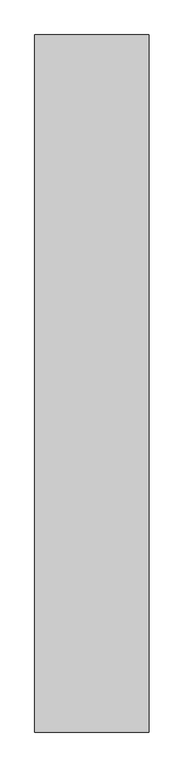
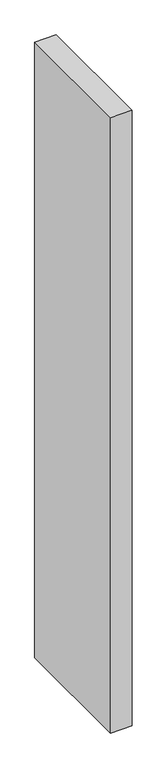
"""IFC4 building model written with IfcOpenShell, lengths in millimetres: proxy geometry, Generic Models 7:Generic Models 1:3:Generic Models 1:3 : Generic Models 7:Generic Models 1:305549:3:Generic Models 1:3:Generic Models 1:3 : Generic Models 7:Generic Models 1:305549:3 : Generic Models 7:Generic Models 1:3:Generic Models 1:3 : Generic Models 7:Generic Models 1:305549:301244:51 : Generic Models 7:Generic Models 1:3:Generic Models 1:3 : Generic Models 7:Generic Models 1:305549:3:Generic Models 1:3:Generic Models 1:3 : Generic Models 7:Generic Models 1:305549:3 : Generic Models 7:Generic Models 1:3:Generic Models 1:3 : Generic Models 7:Generic Models 1:305549:301244:308848."""

from ifc_helpers import new_model, si_unit, origin, origin_with_axes, place, context, project, spatial, polyline, outline, extrude, source, transform, mapped, element, save


def generic_models_49c228d4(model_context):
    return source(origin(), model_context, "Body", "SweptSolid", [
        extrude(outline(polyline([(667344.1117239, -569445.8514763), (667344.1117239, -568206.287148), (667547.3117239, -568206.287148), (667547.3117239, -569445.8514763), (667344.1117239, -569445.8514763)])), origin_with_axes(), (0.0, 0.0, 1.0), 6127.75),
    ])


if __name__ == "__main__":
    model = new_model("IFC4")
    model_context = context("Model", 3, world=origin())
    ifc_project = project(units=[si_unit("LENGTHUNIT", "METRE", prefix="MILLI")], contexts=[model_context])
    site = spatial("IfcSite", under=ifc_project)
    building = spatial("IfcBuilding", under=site)
    placement = place(None, origin())
    generic_models_shape = generic_models_49c228d4(model_context)
    element("IfcBuildingElementProxy", 1, Name="Generic Models 7:Generic Models 1:3:Generic Models 1:3 : Generic Models 7:Generic Models 1:305549:3:Generic Models 1:3:Generic Models 1:3 : Generic Models 7:Generic Models 1:305549:3 : Generic Models 7:Generic Models 1:3:Generic Models 1:3 : Generic Models 7:Generic Models 1:305549:301244:51 : Generic Models 7:Generic Models 1:3:Generic Models 1:3 : Generic Models 7:Generic Models 1:305549:3:Generic Models 1:3:Generic Models 1:3 : Generic Models 7:Generic Models 1:305549:3 : Generic Models 7:Generic Models 1:3:Generic Models 1:3 : Generic Models 7:Generic Models 1:305549:301244:308848", ObjectType="Generic Models 7:Generic Models 1:3:Generic Models 1:3 : Generic Models 7:Generic Models 1:305549:3:Generic Models 1:3:Generic Models 1:3 : Generic Models 7:Generic Models 1:305549:3 : Generic Models 7:Generic Models 1:3:Generic Models 1:3 : Generic Models 7:Generic Models 1:305549:301244:51 : Generic Models 7:Generic Models 1:3:Generic Models 1:3 : Generic Models 7:Generic Models 1:305549:3:Generic Models 1:3:Generic Models 1:3 : Generic Models 7:Generic Models 1:305549:3 : Generic Models 7:Generic Models 1:3:Generic Models 1:3 : Generic Models 7:Generic Models 1:305549:301244:308848", at=placement, inside=building, context=model_context, shape_type="MappedRepresentation", body=[
        mapped(generic_models_shape, transform((0.0, 0.0, 0.0), x_axis=(1.0, 0.0, 0.0), y_axis=(0.0, 1.0, 0.0), z_axis=(0.0, 0.0, 1.0))),
    ])
    save(model, "model.ifc")

# Revit data of these elements
# Type "Generic Models 7:Generic Models 1:3:Generic Models 1:3 : Generic Models 7:Generic Models 1:305549:3:Generic Models 1:3:Generic Models 1:3 : Generic Models 7:Generic Models 1:305549:3 : Generic Models 7:Generic Models 1:3:Generic Models 1:3 : Generic Models 7:Generic Models 1:305549:301244:51 : Generic Models 7:Generic Models 1:3:Generic Models 1:3 : Generic Models 7:Generic Models 1:305549:3:Generic Models 1:3:Generic Models 1:3 : Generic Models 7:Generic Models 1:305549:3 : Generic Models 7:Generic Models 1:3:Generic Models 1:3 : Generic Models 7:Generic Models 1:305549:301244:308848"
#   NameOverride = "Generic Models 7:Generic Models 1:3:Generic Models 1:3 : Generic Models 7:Generic Models 1:305549:3:Generic Models 1:3:Generic Models 1:3 : Generic Models 7:Generic Models 1:305549:3 : Generic Models 7:Generic Models 1:3:Generic Models 1:3 : Generic Models 7:Generic Models 1:305549:301244:308848"
#   ObjectTypeOverride = "Generic Models 1:3:Generic Models 1:3 : Generic Models 7:Generic Models 1:305549:3 : Generic Models 7:Generic Models 1:3:Generic Models 1:3 : Generic Models 7:Generic Models 1:305549:301244"
#   Reference = "Generic Models 1"
#   Tag = "308848"
# Element 1 (IfcBuildingElementProxy, "Generic Models 7:Generic Models 1:3:Generic Models 1:3 : Generic Models 7:Generic Models 1:305549:3:Generic Models 1:3:Generic Models 1:3 : Generic Models 7:Generic Models 1:305549:3 : Generic Models 7:Generic Models 1:3:Generic Models 1:3 : Generic Models 7:Generic Models 1:305549:301244:51 : Generic Models 7:Generic Models 1:3:Generic Models 1:3 : Generic Models 7:Generic Models 1:305549:3:Generic Models 1:3:Generic Models 1:3 : Generic Models 7:Generic Models 1:305549:3 : Generic Models 7:Generic Models 1:3:Generic Models 1:3 : Generic Models 7:Generic Models 1:305549:301244:308848")
#   Materials on its faces: "FULL CAVITY CLASS A FIBERGLASS INSULATION WITH DURABLE VAPOR BARRIER (BLACK) LINER"
# Materials
#   "FULL CAVITY CLASS A FIBERGLASS INSULATION WITH DURABLE VAPOR BARRIER (BLACK) LINER": class "Unassigned", colour RGB 158 92 175, transparency 0, Cost = 0
